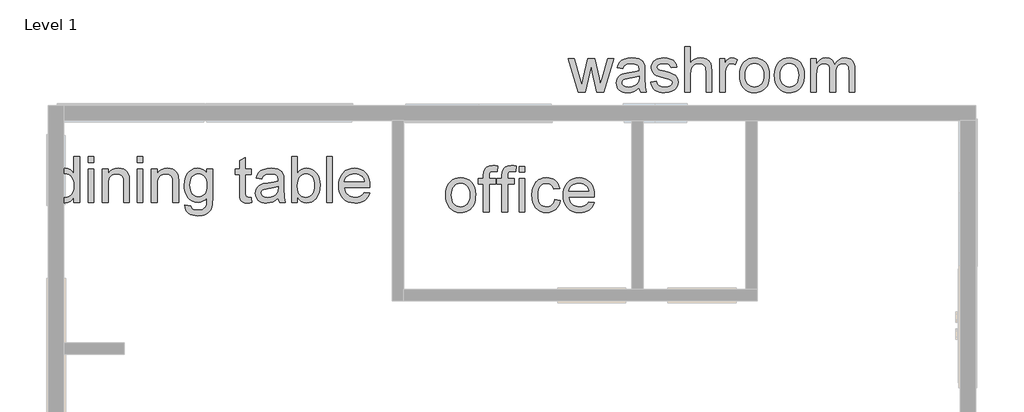
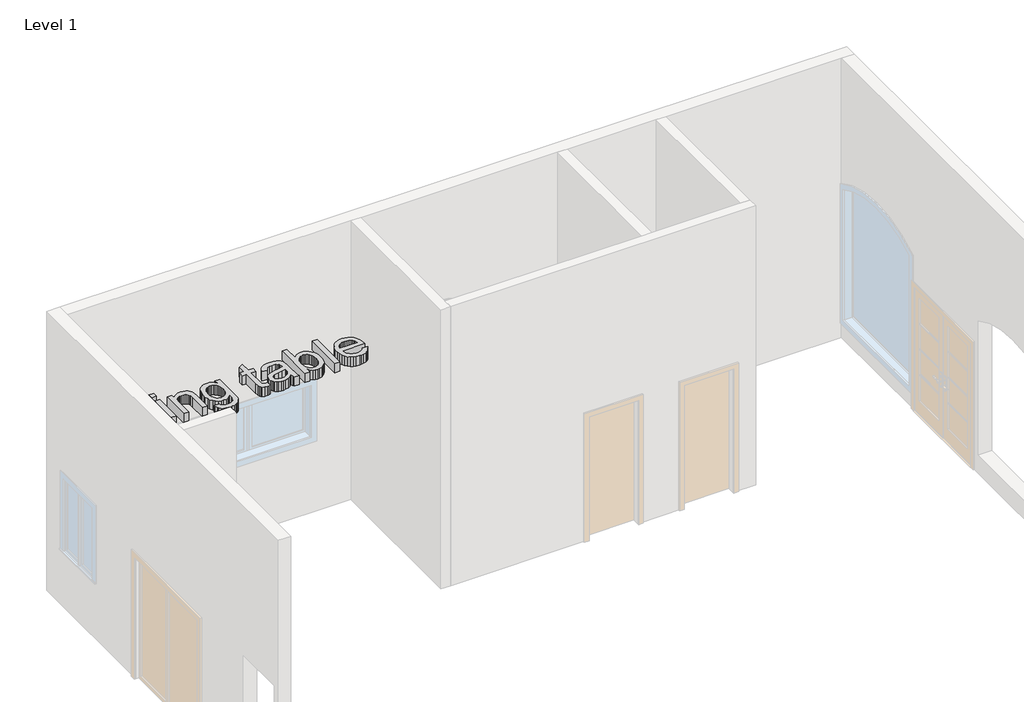
# One storey, part 3 of 3: 3 proxies.
"""IFC4 building model written with IfcOpenShell, lengths in millimetres."""

from ifc_helpers import new_model, si_unit, origin, origin_with_axes, place, context, project, spatial, polyline, outline, extrude, element, save

model = new_model("IFC4")

# Units and contexts
model_context = context("Model", 3, world=origin())
ifc_project = project(units=[si_unit("LENGTHUNIT", "METRE", prefix="MILLI")], contexts=[model_context])

# Site, building, storey
site = spatial("IfcSite", under=ifc_project)
building = spatial("IfcBuilding", under=site)
storey = spatial("IfcBuildingStorey", under=building, Name="Level 1", Elevation=0.0)

# Proxies
placement = place(None, origin())
element("IfcBuildingElementProxy", 1, Name="24\" Arial", ObjectType="24\" Arial", at=placement, inside=storey, context=model_context, shape_type="SweptSolid", body=[
    extrude(outline(polyline([(-71376.3912877, -6229.4340797), (-71512.4649649, -5782.1011603), (-71433.3489034, -5782.1011603), (-71356.1661291, -6043.0949348), (-71333.1153968, -6136.3388645), (-71314.2286679, -6046.515366), (-71252.8096201, -5782.1011603), (-71162.0938352, -5782.1011603), (-71100.9722163, -6045.771794), (-71084.1674889, -6127.1185716), (-71060.0757559, -6041.310362), (-70982.7442671, -5782.1011603), (-70903.3307768, -5782.1011603), (-71040.4454549, -6229.4340797), (-71132.4996694, -6229.4340797), (-71190.9444291, -5967.1018757), (-71207.8978709, -5885.3089549), (-71283.2960724, -6229.4340797), (-71376.3912877, -6229.4340797)])), origin_with_axes(), (0.0, 0.0, 1.0), 152.4),
    extrude(outline(polyline([(-70565.4516568, -6172.3277496), (-70601.8309173, -6203.5205953), (-70639.2883571, -6223.9316469), (-70678.6790842, -6235.1967628), (-70720.8582063, -6238.9518014), (-70754.7604425, -6236.6932015), (-70784.4893808, -6229.9174015), (-70810.0450212, -6218.6244017), (-70831.4273637, -6202.8142019), (-70848.3110956, -6183.4906244), (-70860.3709041, -6161.6574913), (-70867.6067892, -6137.3148027), (-70870.0187509, -6110.4625586), (-70866.3752481, -6078.8979269), (-70855.4447395, -6050.2332261), (-70838.5842443, -6025.6953498), (-70817.1507812, -6006.511192), (-70791.9622795, -5992.0115379), (-70763.8366683, -5981.5271726), (-70697.9561885, -5970.0761637), (-70620.1041993, -5958.0302972), (-70565.8978, -5943.902429), (-70565.4516568, -5926.9489873), (-70570.6938395, -5892.9677466), (-70577.2465678, -5880.3827904), (-70586.4203874, -5870.7349436), (-70602.2770605, -5861.1056861), (-70621.5913433, -5854.227645), (-70670.5927386, -5848.7252122), (-70715.950631, -5852.3873043), (-70747.6267985, -5863.3735807), (-70769.2275653, -5883.6916858), (-70784.3592557, -5915.349264), (-70860.5010292, -5905.8315423), (-70847.2840368, -5864.1915099), (-70827.5607893, -5831.4743416), (-70799.490946, -5806.4531436), (-70761.2341663, -5787.901022), (-70714.4448977, -5776.4128345), (-70660.7775881, -5772.5834386), (-70609.3038159, -5775.9666913), (-70568.500302, -5786.1164492), (-70537.7350103, -5801.3782646), (-70516.3759044, -5820.0976899), (-70502.2108576, -5843.2413686), (-70493.0277433, -5871.7759444), (-70489.3098833, -5938.3999962), (-70489.3098833, -6033.1310699), (-70485.4433089, -6165.4125299), (-70479.7178044, -6198.1111089), (-70470.2744399, -6229.4340797), (-70546.4162134, -6229.4340797), (-70558.6107944, -6202.9629163), (-70565.4516568, -6172.3277496)]), holes=[polyline([(-70565.4516568, -6020.0442026), (-70616.6094109, -6032.7221053), (-70688.2897524, -6043.3923636), (-70753.7984462, -6055.7356589), (-70770.8448345, -6064.1752012), (-70783.4669693, -6075.8121031), (-70791.2744753, -6089.7540782), (-70793.8769774, -6105.1088402), (-70788.2072408, -6127.7506078), (-70771.1980312, -6146.3027294), (-70743.2211344, -6158.6832033), (-70704.6483365, -6162.8100279), (-70663.7518761, -6158.2556494), (-70627.6142766, -6144.5925137), (-70598.3175395, -6124.4603017), (-70577.9436665, -6100.4986937), (-70568.9092666, -6075.8121031), (-70565.8978, -6041.6077908), (-70565.4516568, -6020.0442026)])]), origin_with_axes(), (0.0, 0.0, 1.0), 152.4),
    extrude(outline(polyline([(-70413.1681098, -6096.1859761), (-70337.0263363, -6086.6682544), (-70332.4254845, -6104.0306608), (-70325.0176484, -6119.2367083), (-70314.8028279, -6132.286397), (-70301.7810231, -6143.1797269), (-70285.9150554, -6151.7679836), (-70267.1677462, -6157.9024527), (-70221.0291032, -6162.8100279), (-70175.4481391, -6158.3114173), (-70157.7325361, -6152.688154), (-70143.4001856, -6144.8155853), (-70124.4390995, -6125.2596416), (-70119.6988279, -6114.3105438), (-70118.1187374, -6102.5806953), (-70119.7081226, -6092.3008123), (-70124.4762781, -6083.173466), (-70143.5489, -6068.376383), (-70172.0648865, -6058.7099469), (-70221.9213896, -6046.6640804), (-70291.4081936, -6026.5690469), (-70336.5801931, -6009.4111229), (-70365.5980906, -5990.6916976), (-70386.6225891, -5965.9121605), (-70399.3934384, -5936.652602), (-70403.6503881, -5904.4931127), (-70400.2299569, -5874.9918933), (-70389.9686632, -5847.7585685), (-70373.795972, -5823.8713178), (-70352.6413484, -5804.4083205), (-70331.6168499, -5792.1579717), (-70304.2348108, -5781.8780887), (-70272.5772326, -5774.9071012), (-70238.7261169, -5772.5834386), (-70189.1670427, -5776.319888), (-70146.0770449, -5787.529236), (-70111.4265893, -5805.1147139), (-70087.1861419, -5827.9795532), (-70071.1249866, -5857.8153799), (-70061.0124073, -5896.3138206), (-70137.1541808, -5905.8315423), (-70146.764849, -5881.8699344), (-70165.7817031, -5863.8197239), (-70194.390636, -5852.4988401), (-70232.7775409, -5848.7252122), (-70276.4995749, -5852.3315364), (-70305.6475976, -5863.1505091), (-70322.0433603, -5878.7655212), (-70327.5086146, -5896.7599638), (-70325.24072, -5908.4712229), (-70318.4370361, -5918.9184096), (-70306.8001342, -5928.2502383), (-70290.0325854, -5935.723137), (-70224.4495344, -5951.9330067), (-70157.1748571, -5971.8235579), (-70112.6906618, -5987.7731775), (-70083.1708531, -6004.9125122), (-70060.7893357, -6028.372209), (-70046.6800568, -6058.2266251), (-70041.9769639, -6094.5501177), (-70047.497986, -6132.100504), (-70064.0610525, -6167.4201744), (-70091.034127, -6197.7393229), (-70127.7851735, -6220.2881441), (-70172.1764223, -6234.2858871), (-70222.070104, -6238.9518014), (-70263.0502162, -6236.7024961), (-70298.8439137, -6229.9545801), (-70329.4511964, -6218.7080535), (-70354.8720644, -6202.9629163), (-70375.6363127, -6182.7935256), (-70392.2737364, -6158.2742387), (-70404.7843354, -6129.4050555), (-70413.1681098, -6096.1859761)])), origin_with_axes(), (0.0, 0.0, 1.0), 152.4),
    extrude(outline(polyline([(-69956.3174687, -6229.4340797), (-69956.3174687, -5620.2998916), (-69880.1756952, -5620.2998916), (-69880.1756952, -5844.2637801), (-69852.2080931, -5812.9036307), (-69820.8014704, -5790.503524), (-69785.9558272, -5777.06346), (-69747.6711635, -5772.5834386), (-69701.6812349, -5777.4724246), (-69662.1603827, -5792.1393824), (-69631.0418942, -5815.4317755), (-69619.3585191, -5829.8803091), (-69610.2590566, -5846.1970673), (-69598.5477975, -5888.4691359), (-69594.6440445, -5946.2818595), (-69594.6440445, -6229.4340797), (-69670.785818, -6229.4340797), (-69670.785818, -5954.1637227), (-69672.300846, -5928.4547206), (-69676.8459298, -5906.5007571), (-69684.4210697, -5888.3018322), (-69695.0262654, -5873.857946), (-69708.4105615, -5862.8623749), (-69724.3230025, -5855.0083956), (-69742.7635883, -5850.296008), (-69763.7323189, -5848.7252122), (-69795.9103975, -5852.9635726), (-69826.1180103, -5865.6786539), (-69851.1392083, -5885.6435623), (-69867.7580426, -5911.6314039), (-69877.071282, -5946.1703237), (-69880.1756952, -5991.7884663), (-69880.1756952, -6229.4340797), (-69956.3174687, -6229.4340797)])), origin_with_axes(), (0.0, 0.0, 1.0), 152.4),
    extrude(outline(polyline([(-69489.9491059, -6229.4340797), (-69489.9491059, -5782.1011603), (-69423.3250541, -5782.1011603), (-69423.3250541, -5848.2790689), (-69398.7128206, -5809.9107534), (-69376.0338744, -5787.3061644), (-69353.280571, -5776.2641201), (-69328.445266, -5772.5834386), (-69290.5230936, -5778.4576575), (-69252.0060636, -5796.0803141), (-69277.4362263, -5864.3402243), (-69304.2048185, -5852.6289652), (-69330.9734108, -5848.7252122), (-69353.7081249, -5852.4802508), (-69374.02623, -5863.7453667), (-69390.4405821, -5881.6654521), (-69401.4640371, -5905.3853991), (-69410.7215085, -5947.9177179), (-69413.8073324, -5994.3166111), (-69413.8073324, -6229.4340797), (-69489.9491059, -6229.4340797)])), origin_with_axes(), (0.0, 0.0, 1.0), 152.4),
    extrude(outline(polyline([(-69223.4528986, -6005.76762), (-69219.3353686, -5947.834066), (-69206.9827786, -5897.9125004), (-69186.3951287, -5856.0029232), (-69157.5724188, -5822.1053343), (-69128.5545212, -5800.4395049), (-69096.525157, -5784.9639126), (-69061.4843262, -5775.6785571), (-69023.4320287, -5772.5834386), (-68981.4248576, -5776.3524192), (-68943.44227, -5787.6593611), (-68909.4842659, -5806.5042641), (-68879.5508453, -5832.8871284), (-68855.1198576, -5865.9156675), (-68837.669152, -5904.697595), (-68827.1987287, -5949.2329109), (-68823.7085876, -5999.5216152), (-68825.2514995, -6040.2786558), (-68829.8802353, -6076.4441393), (-68837.5947948, -6108.0180656), (-68848.3951782, -6135.0004348), (-68862.1466131, -6158.3067699), (-68878.7143268, -6178.852594), (-68898.0983196, -6196.6379069), (-68920.2985913, -6211.6627088), (-68944.4507396, -6223.6016868), (-68969.6903619, -6232.1295283), (-68996.0174583, -6237.2462331), (-69023.4320287, -6238.9518014), (-69066.0526467, -6235.1967628), (-69104.388431, -6223.9316469), (-69138.4393816, -6205.1564537), (-69168.2054985, -6178.8711833), (-69192.376236, -6145.5219787), (-69209.6410485, -6105.5549834), (-69219.9999361, -6058.9701971), (-69223.4528986, -6005.76762)]), holes=[polyline([(-69147.3111251, -6005.6189056), (-69145.108293, -6042.5511978), (-69138.4997968, -6074.5294414), (-69127.4856364, -6101.5536365), (-69112.0658119, -6123.6237831), (-69093.3092081, -6140.7677652), (-69072.2847096, -6153.0134667), (-69048.9923164, -6160.3608876), (-69023.4320287, -6162.8100279), (-68998.0018661, -6160.3469456), (-68974.8024194, -6152.9576988), (-68953.8336888, -6140.6422875), (-68935.0956743, -6123.4007115), (-68919.6758498, -6101.1121406), (-68908.6616894, -6073.6557443), (-68902.0531932, -6041.0315225), (-68899.8503611, -6003.2394752), (-68902.0671352, -5967.478309), (-68908.7174573, -5936.3365839), (-68919.8013275, -5909.8142999), (-68935.3187459, -5887.9114569), (-68954.1264703, -5870.7674748), (-68975.0812589, -5858.5217733), (-68998.1831117, -5851.1743525), (-69023.4320287, -5848.7252122), (-69048.9923164, -5851.1650578), (-69072.2847096, -5858.4845947), (-69093.3092081, -5870.683823), (-69112.0658119, -5887.7627425), (-69127.4856364, -5909.7678266), (-69138.4997968, -5936.7455485), (-69145.108293, -5968.6959082), (-69147.3111251, -6005.6189056)])]), origin_with_axes(), (0.0, 0.0, 1.0), 152.4),
    extrude(outline(polyline([(-68757.0845358, -6005.76762), (-68752.9670058, -5947.834066), (-68740.6144158, -5897.9125004), (-68720.0267659, -5856.0029232), (-68691.204056, -5822.1053343), (-68662.1861584, -5800.4395049), (-68630.1567942, -5784.9639126), (-68595.1159634, -5775.6785571), (-68557.0636659, -5772.5834386), (-68515.0564948, -5776.3524192), (-68477.0739072, -5787.6593611), (-68443.1159032, -5806.5042641), (-68413.1824825, -5832.8871284), (-68388.7514948, -5865.9156675), (-68371.3007893, -5904.697595), (-68360.8303659, -5949.2329109), (-68357.3402248, -5999.5216152), (-68358.8831367, -6040.2786558), (-68363.5118725, -6076.4441393), (-68371.2264321, -6108.0180656), (-68382.0268155, -6135.0004348), (-68395.7782503, -6158.3067699), (-68412.345964, -6178.852594), (-68431.7299568, -6196.6379069), (-68453.9302285, -6211.6627088), (-68478.0823768, -6223.6016868), (-68503.3219991, -6232.1295283), (-68529.6490955, -6237.2462331), (-68557.0636659, -6238.9518014), (-68599.6842839, -6235.1967628), (-68638.0200682, -6223.9316469), (-68672.0710188, -6205.1564537), (-68701.8371357, -6178.8711833), (-68726.0078732, -6145.5219787), (-68743.2726858, -6105.5549834), (-68753.6315733, -6058.9701971), (-68757.0845358, -6005.76762)]), holes=[polyline([(-68680.9427623, -6005.6189056), (-68678.7399302, -6042.5511978), (-68672.131434, -6074.5294414), (-68661.1172736, -6101.5536365), (-68645.6974491, -6123.6237831), (-68626.9408453, -6140.7677652), (-68605.9163468, -6153.0134667), (-68582.6239536, -6160.3608876), (-68557.0636659, -6162.8100279), (-68531.6335033, -6160.3469456), (-68508.4340566, -6152.9576988), (-68487.465326, -6140.6422875), (-68468.7273115, -6123.4007115), (-68453.307487, -6101.1121406), (-68442.2933266, -6073.6557443), (-68435.6848304, -6041.0315225), (-68433.4819983, -6003.2394752), (-68435.6987724, -5967.478309), (-68442.3490945, -5936.3365839), (-68453.4329648, -5909.8142999), (-68468.9503831, -5887.9114569), (-68487.7581075, -5870.7674748), (-68508.7128961, -5858.5217733), (-68531.8147489, -5851.1743525), (-68557.0636659, -5848.7252122), (-68582.6239536, -5851.1650578), (-68605.9163468, -5858.4845947), (-68626.9408453, -5870.683823), (-68645.6974491, -5887.7627425), (-68661.1172736, -5909.7678266), (-68672.131434, -5936.7455485), (-68678.7399302, -5968.6959082), (-68680.9427623, -6005.6189056)])]), origin_with_axes(), (0.0, 0.0, 1.0), 152.4),
    extrude(outline(polyline([(-68271.6807296, -6229.4340797), (-68271.6807296, -5782.1011603), (-68195.5389561, -5782.1011603), (-68195.5389561, -5855.714789), (-68172.6369383, -5821.900852), (-68143.1914868, -5795.4110993), (-68108.2064239, -5778.2903538), (-68068.6855717, -5772.5834386), (-68026.3391459, -5778.4018896), (-68008.3168194, -5785.6749533), (-67992.3950838, -5795.8572425), (-67978.6204124, -5808.660623), (-67967.0392783, -5823.7969606), (-67950.4576226, -5861.0685075), (-67922.7037974, -5822.3562899), (-67891.0462192, -5794.7047058), (-67855.484888, -5778.1137554), (-67816.0198037, -5772.5834386), (-67785.5379988, -5774.8838645), (-67758.7833485, -5781.7851422), (-67735.7558529, -5793.2872717), (-67716.455512, -5809.390253), (-67701.1983439, -5830.2799791), (-67690.3003666, -5856.1423429), (-67683.7615803, -5886.9773446), (-67681.5819849, -5922.7849841), (-67681.5819849, -6229.4340797), (-67757.7237584, -6229.4340797), (-67757.7237584, -5955.5021524), (-67759.4897419, -5917.5242121), (-67764.7876924, -5891.9267458), (-67774.7143787, -5874.3970357), (-67790.3665695, -5860.6223643), (-67810.4987816, -5851.6995002), (-67833.8655319, -5848.7252122), (-67855.4430621, -5850.6306154), (-67875.115189, -5856.3468252), (-67892.8819126, -5865.8738416), (-67908.743233, -5879.2116644), (-67921.7882744, -5896.7506692), (-67931.1061611, -5918.881231), (-67936.6968931, -5945.60335), (-67938.5604705, -5976.9170262), (-67938.5604705, -6229.4340797), (-68014.702244, -6229.4340797), (-68014.702244, -5947.0254315), (-68019.1079081, -5903.9726123), (-68024.6149883, -5887.0749384), (-68032.3249006, -5873.2630884), (-68042.5443683, -5862.5277675), (-68055.5801151, -5854.8596812), (-68071.4321408, -5850.2588294), (-68090.1004455, -5848.7252122), (-68119.4343612, -5852.8148582), (-68146.4632036, -5865.0837963), (-68168.7703638, -5885.2345977), (-68183.9392328, -5912.9698336), (-68192.6390253, -5951.4496849), (-68195.5389561, -6003.8343328), (-68195.5389561, -6229.4340797), (-68271.6807296, -6229.4340797)])), origin_with_axes(), (0.0, 0.0, 1.0), 152.4),
])
element("IfcBuildingElementProxy", 2, Name="24\" Arial", ObjectType="24\" Arial", at=placement, inside=storey, context=model_context, shape_type="SweptSolid", body=[
    extrude(outline(polyline([(-73151.8600009, -7609.8505265), (-73147.742471, -7551.9169725), (-73135.389881, -7501.9954069), (-73114.802231, -7460.0858296), (-73085.9795211, -7426.1882408), (-73056.9616235, -7404.5224114), (-73024.9322593, -7389.046819), (-72989.8914285, -7379.7614636), (-72951.8391311, -7376.6663451), (-72909.83196, -7380.4353257), (-72871.8493724, -7391.7422675), (-72837.8913683, -7410.5871706), (-72807.9579477, -7436.9700349), (-72783.5269599, -7469.998574), (-72766.0762544, -7508.7805014), (-72755.6058311, -7553.3158173), (-72752.11569, -7603.6045216), (-72753.6586019, -7644.3615623), (-72758.2873376, -7680.5270458), (-72766.0018972, -7712.1009721), (-72776.8022806, -7739.0833413), (-72790.5537154, -7762.3896764), (-72807.1214292, -7782.9355004), (-72826.505422, -7800.7208134), (-72848.7056937, -7815.7456152), (-72872.8578419, -7827.6845933), (-72898.0974642, -7836.2124347), (-72924.4245606, -7841.3291396), (-72951.8391311, -7843.0347079), (-72994.459749, -7839.2796693), (-73032.7955333, -7828.0145534), (-73066.8464839, -7809.2393602), (-73096.6126008, -7782.9540897), (-73120.7833384, -7749.6048852), (-73138.0481509, -7709.6378898), (-73148.4070384, -7663.0531036), (-73151.8600009, -7609.8505265)]), holes=[polyline([(-73075.7182274, -7609.7018121), (-73073.5153954, -7646.6341042), (-73066.9068991, -7678.6123478), (-73055.8927388, -7705.636543), (-73040.4729143, -7727.7066896), (-73021.7163104, -7744.8506717), (-73000.6918119, -7757.0963732), (-72977.3994188, -7764.4437941), (-72951.8391311, -7766.8929344), (-72926.4089684, -7764.4298521), (-72903.2095218, -7757.0406053), (-72882.2407912, -7744.7251939), (-72863.5027766, -7727.483618), (-72848.0829521, -7705.1950471), (-72837.0687918, -7677.7386507), (-72830.4602956, -7645.1144289), (-72828.2574635, -7607.3223817), (-72830.4742375, -7571.5612155), (-72837.1245597, -7540.4194903), (-72848.2084299, -7513.8972063), (-72863.7258482, -7491.9943634), (-72882.5335727, -7474.8503813), (-72903.4883613, -7462.6046798), (-72926.5902141, -7455.2572589), (-72951.8391311, -7452.8081186), (-72977.3994188, -7455.2479643), (-73000.6918119, -7462.5675012), (-73021.7163104, -7474.7667295), (-73040.4729143, -7491.845649), (-73055.8927388, -7513.8507331), (-73066.9068991, -7540.8284549), (-73073.5153954, -7572.7788146), (-73075.7182274, -7609.7018121)])]), origin_with_axes(), (0.0, 0.0, 1.0), 152.4),
    extrude(outline(polyline([(-72647.4207514, -7833.5169862), (-72647.4207514, -7462.3258403), (-72714.0448032, -7462.3258403), (-72714.0448032, -7386.1840668), (-72647.4207514, -7386.1840668), (-72647.4207514, -7341.1236032), (-72645.413107, -7303.833467), (-72639.3901737, -7277.6225538), (-72624.0725904, -7252.3039269), (-72600.4270005, -7232.2646613), (-72567.3380462, -7219.2149726), (-72523.6903694, -7214.8650764), (-72490.6385937, -7216.947078), (-72454.240744, -7223.1930829), (-72465.3943241, -7294.5759955), (-72509.2650725, -7291.0068499), (-72538.2086129, -7294.1670309), (-72557.2254669, -7303.647574), (-72567.7656001, -7321.7535524), (-72571.2789779, -7350.7900393), (-72571.2789779, -7386.1840668), (-72485.6194827, -7386.1840668), (-72485.6194827, -7462.3258403), (-72571.2789779, -7462.3258403), (-72571.2789779, -7833.5169862), (-72647.4207514, -7833.5169862)])), origin_with_axes(), (0.0, 0.0, 1.0), 152.4),
    extrude(outline(polyline([(-72399.9599875, -7833.5169862), (-72399.9599875, -7462.3258403), (-72466.5840393, -7462.3258403), (-72466.5840393, -7386.1840668), (-72399.9599875, -7386.1840668), (-72399.9599875, -7341.1236032), (-72397.952343, -7303.833467), (-72391.9294098, -7277.6225538), (-72376.6118264, -7252.3039269), (-72352.9662366, -7232.2646613), (-72319.8772823, -7219.2149726), (-72276.2296055, -7214.8650764), (-72243.1778298, -7216.947078), (-72206.77998, -7223.1930829), (-72217.9335601, -7294.5759955), (-72261.8043086, -7291.0068499), (-72290.7478489, -7294.1670309), (-72309.764703, -7303.647574), (-72320.3048362, -7321.7535524), (-72323.8182139, -7350.7900393), (-72323.8182139, -7386.1840668), (-72238.1587187, -7386.1840668), (-72238.1587187, -7462.3258403), (-72323.8182139, -7462.3258403), (-72323.8182139, -7833.5169862), (-72399.9599875, -7833.5169862)])), origin_with_axes(), (0.0, 0.0, 1.0), 152.4),
    extrude(outline(polyline([(-72171.5346669, -7833.5169862), (-72171.5346669, -7386.1840668), (-72095.3928934, -7386.1840668), (-72095.3928934, -7833.5169862), (-72171.5346669, -7833.5169862)])), origin_with_axes(), (0.0, 0.0, 1.0), 152.4),
    extrude(outline(polyline([(-72171.5346669, -7300.5245716), (-72171.5346669, -7224.3827981), (-72095.3928934, -7224.3827981), (-72095.3928934, -7300.5245716), (-72171.5346669, -7300.5245716)])), origin_with_axes(), (0.0, 0.0, 1.0), 152.4),
    extrude(outline(polyline([(-71695.6485824, -7671.7157175), (-71619.5068089, -7681.2334392), (-71627.7883421, -7717.1619091), (-71640.7357897, -7748.9542597), (-71658.3491516, -7776.610491), (-71680.6284279, -7800.1306031), (-71706.6348588, -7818.9011489), (-71735.4296848, -7832.3086817), (-71767.0129058, -7840.3532013), (-71801.3845218, -7843.0347079), (-71844.0887916, -7839.2936112), (-71882.3781027, -7828.0703213), (-71916.2524549, -7809.364838), (-71945.7118484, -7783.1771613), (-71969.5572732, -7749.9999078), (-71986.5897195, -7710.3256939), (-71996.8091872, -7664.1545196), (-72000.2156765, -7611.4863849), (-71994.3972255, -7543.7283858), (-71987.1241618, -7513.2372862), (-71976.9418727, -7485.0047865), (-71963.7806482, -7459.5978605), (-71947.5707784, -7437.5834818), (-71928.3122634, -7418.9616503), (-71906.0051032, -7403.7323662), (-71881.6577673, -7391.8909819), (-71856.2787252, -7383.4328504), (-71829.867977, -7378.3579714), (-71802.4255226, -7376.6663451), (-71768.6441169, -7378.9900076), (-71738.0879547, -7385.9609952), (-71710.7570361, -7397.5793078), (-71686.6513611, -7413.8449455), (-71666.1798943, -7434.3861221), (-71649.7516003, -7458.8310519), (-71637.3664791, -7487.1797346), (-71629.0245306, -7519.4321704), (-71705.1663041, -7528.9498921), (-71718.9781541, -7495.7308127), (-71740.4859744, -7471.9179192), (-71768.5000498, -7457.5855688), (-71801.830665, -7452.8081186), (-71827.7023235, -7455.1596651), (-71851.0365426, -7462.2143045), (-71871.8333222, -7473.9720369), (-71890.0926623, -7490.4328622), (-71904.9594551, -7511.9778611), (-71915.5785928, -7538.9881142), (-71921.9500754, -7571.4636216), (-71924.073903, -7609.4043833), (-71921.9965487, -7647.9167659), (-71915.7644858, -7680.7687067), (-71905.3777143, -7707.9602055), (-71890.8362343, -7729.4912624), (-71872.9393855, -7745.8544939), (-71852.486508, -7757.5425164), (-71829.4776017, -7764.5553299), (-71803.9126666, -7766.8929344), (-71764.484761, -7761.0558941), (-71747.4337254, -7753.7595938), (-71732.157968, -7743.5447734), (-71719.0850426, -7730.299897), (-71708.6425032, -7713.9134289), (-71700.8303498, -7694.385369), (-71695.6485824, -7671.7157175)])), origin_with_axes(), (0.0, 0.0, 1.0), 152.4),
    extrude(outline(polyline([(-71239.6902277, -7700.2688826), (-71165.0355982, -7709.7866042), (-71176.4819598, -7739.6874936), (-71191.9343156, -7766.0378266), (-71211.3926655, -7788.8376032), (-71234.8570097, -7808.0868236), (-71262.0856871, -7823.376523), (-71292.8370369, -7834.2977368), (-71327.1110591, -7840.8504651), (-71364.9077537, -7843.0347079), (-71412.1524601, -7839.2657273), (-71454.2479304, -7827.9587855), (-71491.1941644, -7809.1138824), (-71522.9911624, -7782.7310181), (-71548.5607448, -7749.54447), (-71566.8247322, -7710.2885153), (-71577.7831247, -7664.9631542), (-71581.4359221, -7613.5683865), (-71577.7459461, -7560.430872), (-71566.6760178, -7513.5951302), (-71548.2261374, -7473.0611612), (-71522.3963048, -7438.8289649), (-71490.6829587, -7411.6328187), (-71454.5825378, -7392.207), (-71414.095042, -7380.5515088), (-71369.2204714, -7376.6663451), (-71325.7912188, -7380.5422142), (-71286.5166749, -7392.1698214), (-71251.3968395, -7411.5491669), (-71220.4317127, -7438.6802505), (-71195.1549118, -7472.8380896), (-71177.100054, -7513.2977014), (-71166.2671394, -7560.059086), (-71162.6561678, -7613.1222433), (-71163.102311, -7633.6448307), (-71505.2941486, -7633.6448307), (-71500.8838372, -7664.0290419), (-71492.1143348, -7690.6396251), (-71478.9856416, -7713.4765803), (-71461.4977574, -7732.5399077), (-71440.617326, -7747.5693568), (-71417.3109909, -7758.3046777), (-71391.5787521, -7764.7458702), (-71363.4206097, -7766.8929344), (-71322.8959353, -7762.9148241), (-71288.7659802, -7750.9804934), (-71261.0307443, -7730.3463702), (-71239.6902277, -7700.2688826)]), holes=[polyline([(-71505.2941486, -7557.5030572), (-71238.7979413, -7557.5030572), (-71249.0964136, -7517.2758116), (-71257.9542152, -7501.4563172), (-71269.2843936, -7488.499575), (-71290.0486419, -7472.8845628), (-71313.6756424, -7461.7309827), (-71340.1653952, -7455.0388346), (-71369.5179002, -7452.8081186), (-71396.2911397, -7454.5880441), (-71420.8429579, -7459.9278206), (-71443.1733548, -7468.827448), (-71463.2823302, -7481.2869265), (-71480.1567675, -7496.7299876), (-71492.7835496, -7514.5803631), (-71501.1626767, -7534.838053), (-71505.2941486, -7557.5030572)])]), origin_with_axes(), (0.0, 0.0, 1.0), 152.4),
])
element("IfcBuildingElementProxy", 3, Name="24\" Arial", ObjectType="24\" Arial", at=placement, inside=storey, context=model_context, shape_type="SweptSolid", body=[
    extrude(outline(polyline([(-78123.1451861, -7705.9587097), (-78123.1451861, -7634.1296538), (-78145.9263735, -7669.718869), (-78173.5221896, -7695.139737), (-78205.9326345, -7710.3922578), (-78243.1577081, -7715.4764314), (-78268.2904419, -7713.6360907), (-78292.3821749, -7708.1150685), (-78315.4329072, -7698.913365), (-78337.4426386, -7686.0309799), (-78357.7235651, -7669.8536415), (-78375.5878825, -7650.7670775), (-78391.035591, -7628.7712881), (-78404.0666904, -7603.8662732), (-78414.4116359, -7576.5260599), (-78421.8008828, -7547.2246755), (-78427.7122802, -7482.7383932), (-78422.2656153, -7419.0514508), (-78405.9256204, -7361.5361561), (-78393.6752716, -7335.9108058), (-78378.710885, -7313.4642258), (-78361.0324605, -7294.1964162), (-78340.6399982, -7278.1073769), (-78318.2538335, -7265.4201795), (-78294.5943017, -7256.3578957), (-78269.6614028, -7250.9205254), (-78243.4551369, -7249.1080686), (-78206.2021793, -7254.2944834), (-78173.2619394, -7269.8537276), (-78145.3408106, -7293.7037997), (-78123.1451861, -7323.7626981), (-78123.1451861, -7096.8245216), (-78047.0034126, -7096.8245216), (-78047.0034126, -7705.9587097), (-78123.1451861, -7705.9587097)]), holes=[polyline([(-78351.5705067, -7482.4409644), (-78349.4234425, -7519.3639619), (-78342.98225, -7551.3143216), (-78332.2469292, -7578.2920434), (-78317.21748, -7600.2971275), (-78299.2695107, -7617.3760471), (-78279.7786294, -7629.5752753), (-78258.7448363, -7636.8948122), (-78236.1681312, -7639.3346579), (-78213.4845377, -7637.006348), (-78192.5762223, -7630.0214185), (-78173.4431851, -7618.3798693), (-78156.0854261, -7602.0817003), (-78141.6740711, -7580.9967866), (-78131.3802461, -7554.995003), (-78125.2039511, -7524.0763495), (-78123.1451861, -7488.2408261), (-78125.2411297, -7448.9523402), (-78131.5289605, -7415.2592336), (-78142.0086785, -7387.1615064), (-78156.6802837, -7364.6591585), (-78174.4191234, -7347.4175826), (-78194.1005449, -7335.1021712), (-78215.7245483, -7327.7129244), (-78239.2911336, -7325.2498421), (-78262.3139819, -7327.6153306), (-78283.3477751, -7334.7117959), (-78302.3925131, -7346.5392382), (-78319.448196, -7363.0976573), (-78333.5017069, -7384.7495447), (-78343.539929, -7411.8573917), (-78349.5628623, -7444.4211982), (-78351.5705067, -7482.4409644)])]), origin_with_axes(), (0.0, 0.0, 1.0), 152.4),
    extrude(outline(polyline([(-77932.7907524, -7705.9587097), (-77932.7907524, -7258.6257903), (-77856.6489788, -7258.6257903), (-77856.6489788, -7705.9587097), (-77932.7907524, -7705.9587097)])), origin_with_axes(), (0.0, 0.0, 1.0), 152.4),
    extrude(outline(polyline([(-77932.7907524, -7172.9662951), (-77932.7907524, -7096.8245216), (-77856.6489788, -7096.8245216), (-77856.6489788, -7172.9662951), (-77932.7907524, -7172.9662951)])), origin_with_axes(), (0.0, 0.0, 1.0), 152.4),
    extrude(outline(polyline([(-77742.4363186, -7705.9587097), (-77742.4363186, -7258.6257903), (-77666.294545, -7258.6257903), (-77666.294545, -7321.0858389), (-77639.8419709, -7289.5955644), (-77608.0728569, -7267.1025112), (-77570.987203, -7253.6066793), (-77528.5850093, -7249.1080686), (-77491.0532123, -7252.7329822), (-77456.6815963, -7263.6077228), (-77428.0168954, -7280.3752715), (-77407.6058438, -7301.6786095), (-77393.7568152, -7327.4619689), (-77384.7781832, -7357.6695816), (-77380.7628944, -7431.2832103), (-77380.7628944, -7705.9587097), (-77456.9046679, -7705.9587097), (-77456.9046679, -7441.544504), (-77459.0982053, -7402.1723663), (-77465.6788176, -7374.1768802), (-77477.8176306, -7354.1190253), (-77496.6857702, -7338.5597811), (-77520.8704498, -7328.5773269), (-77548.9588823, -7325.2498421), (-77572.0793244, -7327.1180668), (-77593.5546135, -7332.7227408), (-77613.3847494, -7342.0638641), (-77631.5697323, -7355.1414368), (-77646.7618379, -7373.4426028), (-77657.6133419, -7398.4545062), (-77664.1242442, -7430.177147), (-77666.294545, -7468.6105251), (-77666.294545, -7705.9587097), (-77742.4363186, -7705.9587097)])), origin_with_axes(), (0.0, 0.0, 1.0), 152.4),
    extrude(outline(polyline([(-77276.0679558, -7705.9587097), (-77276.0679558, -7258.6257903), (-77199.9261823, -7258.6257903), (-77199.9261823, -7705.9587097), (-77276.0679558, -7705.9587097)])), origin_with_axes(), (0.0, 0.0, 1.0), 152.4),
    extrude(outline(polyline([(-77276.0679558, -7172.9662951), (-77276.0679558, -7096.8245216), (-77199.9261823, -7096.8245216), (-77199.9261823, -7172.9662951), (-77276.0679558, -7172.9662951)])), origin_with_axes(), (0.0, 0.0, 1.0), 152.4),
    extrude(outline(polyline([(-77085.713522, -7705.9587097), (-77085.713522, -7258.6257903), (-77009.5717485, -7258.6257903), (-77009.5717485, -7321.0858389), (-76983.1191743, -7289.5955644), (-76951.3500603, -7267.1025112), (-76914.2644065, -7253.6066793), (-76871.8622128, -7249.1080686), (-76834.3304157, -7252.7329822), (-76799.9587997, -7263.6077228), (-76771.2940988, -7280.3752715), (-76750.8830472, -7301.6786095), (-76737.0340186, -7327.4619689), (-76728.0553866, -7357.6695816), (-76724.0400978, -7431.2832103), (-76724.0400978, -7705.9587097), (-76800.1818713, -7705.9587097), (-76800.1818713, -7441.544504), (-76802.3754087, -7402.1723663), (-76808.956021, -7374.1768802), (-76821.094834, -7354.1190253), (-76839.9629737, -7338.5597811), (-76864.1476532, -7328.5773269), (-76892.2360858, -7325.2498421), (-76915.3565278, -7327.1180668), (-76936.8318169, -7332.7227408), (-76956.6619528, -7342.0638641), (-76974.8469357, -7355.1414368), (-76990.0390413, -7373.4426028), (-77000.8905453, -7398.4545062), (-77007.4014477, -7430.177147), (-77009.5717485, -7468.6105251), (-77009.5717485, -7705.9587097), (-77085.713522, -7705.9587097)])), origin_with_axes(), (0.0, 0.0, 1.0), 152.4),
    extrude(outline(polyline([(-76638.3806026, -7744.0295965), (-76562.238829, -7753.5473182), (-76553.8364654, -7777.3416224), (-76537.5522384, -7793.7002066), (-76505.5414635, -7806.4152879), (-76463.6411809, -7810.6536483), (-76418.9525033, -7805.8576089), (-76400.9022928, -7799.8625596), (-76385.7148346, -7791.4694905), (-76362.6641024, -7768.4187583), (-76348.5362342, -7737.6348772), (-76344.4094096, -7704.8805303), (-76343.3312302, -7648.8523796), (-76368.6684463, -7673.836399), (-76396.9427719, -7691.6821272), (-76428.1542069, -7702.3895641), (-76462.3027513, -7705.9587097), (-76504.0496722, -7701.8040011), (-76540.8053659, -7689.3398754), (-76572.5698326, -7668.5663324), (-76599.3430722, -7639.4833723), (-76620.585995, -7604.5912559), (-76635.7595112, -7566.390244), (-76644.863621, -7524.8803367), (-76647.8983243, -7480.061534), (-76642.4516593, -7418.5867183), (-76626.1116644, -7362.0566565), (-76614.0007354, -7336.5660786), (-76599.454608, -7314.1520299), (-76582.4732823, -7294.8145104), (-76563.0567583, -7278.5535201), (-76541.5164067, -7265.6711351), (-76518.1635983, -7256.4694315), (-76492.9983332, -7250.9484093), (-76466.0206113, -7249.1080686), (-76430.4128069, -7253.2720719), (-76398.0953085, -7265.7640816), (-76369.0681163, -7286.5840978), (-76343.3312302, -7315.7321204), (-76343.3312302, -7258.6257903), (-76267.1894567, -7258.6257903), (-76267.1894567, -7644.8370907), (-76272.3944607, -7734.0099637), (-76278.9007158, -7767.1779225), (-76288.0094729, -7792.7335629), (-76299.9391563, -7813.3444495), (-76314.9081902, -7831.6781468), (-76332.9165748, -7847.7346548), (-76353.9643099, -7861.5139736), (-76377.8376186, -7872.5746072), (-76404.3227241, -7880.4750598), (-76433.4196262, -7885.2153313), (-76465.1283249, -7886.7954218), (-76502.4324031, -7884.5693531), (-76535.9721479, -7877.891147), (-76565.7475595, -7866.7608036), (-76591.7586377, -7851.1783227), (-76612.7691942, -7831.1251151), (-76627.5430406, -7806.5825916), (-76636.0801767, -7777.550752), (-76638.3806026, -7744.0295965)]), holes=[polyline([(-76571.7565507, -7474.8565299), (-76569.7256697, -7512.5045101), (-76563.6330266, -7544.6965307), (-76553.4786213, -7571.4325917), (-76539.262454, -7592.7126931), (-76521.9790522, -7608.9457994), (-76502.6229434, -7620.5408754), (-76481.1941276, -7627.497921), (-76457.6926049, -7629.8169362), (-76434.4234484, -7627.511863), (-76413.0968737, -7620.5966433), (-76393.712881, -7609.0712772), (-76376.2714701, -7592.9357647), (-76361.8601151, -7571.8647929), (-76351.5662902, -7545.5330492), (-76345.3899952, -7513.9405336), (-76343.3312302, -7477.087246), (-76345.4504104, -7441.772223), (-76351.8079511, -7411.076641), (-76362.4038522, -7385.0005002), (-76377.2381137, -7363.5438005), (-76395.0559579, -7346.7901937), (-76414.6026071, -7334.8233317), (-76435.8780611, -7327.6432145), (-76458.8823201, -7325.2498421), (-76481.5008511, -7327.6060359), (-76502.3626932, -7334.6746173), (-76521.4678464, -7346.4555863), (-76538.8163108, -7362.9489429), (-76553.2276658, -7384.0803299), (-76563.5214908, -7409.77539), (-76569.6977857, -7440.0341234), (-76571.7565507, -7474.8565299)])]), origin_with_axes(), (0.0, 0.0, 1.0), 152.4),
    extrude(outline(polyline([(-75753.2324854, -7642.4576603), (-75743.7147637, -7708.1894257), (-75773.8666086, -7713.65468), (-75800.6723795, -7715.4764314), (-75837.2189436, -7712.3162504), (-75864.4708577, -7702.8357073), (-75883.7293727, -7688.2245174), (-75896.2957396, -7669.6723958), (-75903.2109592, -7637.8103353), (-75905.5160325, -7583.2693286), (-75905.5160325, -7334.7675638), (-75962.6223626, -7334.7675638), (-75962.6223626, -7258.6257903), (-75905.5160325, -7258.6257903), (-75905.5160325, -7149.9155629), (-75829.3742589, -7105.1525281), (-75829.3742589, -7258.6257903), (-75753.2324854, -7258.6257903), (-75753.2324854, -7334.7675638), (-75829.3742589, -7334.7675638), (-75829.3742589, -7581.0386125), (-75825.3589701, -7620.2992145), (-75812.34646, -7634.204011), (-75801.3601836, -7638.0519962), (-75786.3957969, -7639.3346579), (-75753.2324854, -7642.4576603)])), origin_with_axes(), (0.0, 0.0, 1.0), 152.4),
    extrude(outline(polyline([(-75391.5590612, -7648.8523796), (-75427.9383217, -7680.0452253), (-75465.3957615, -7700.4562769), (-75504.7864886, -7711.7213928), (-75546.9656107, -7715.4764314), (-75580.8678469, -7713.2178314), (-75610.5967852, -7706.4420315), (-75636.1524256, -7695.1490317), (-75657.5347681, -7679.3388319), (-75674.4185, -7660.0152543), (-75686.4783085, -7638.1821213), (-75693.7141936, -7613.8394327), (-75696.1261553, -7586.9871886), (-75692.4826525, -7555.4225569), (-75681.552144, -7526.757856), (-75664.6916487, -7502.2199798), (-75643.2581856, -7483.035822), (-75618.0696839, -7468.5361679), (-75589.9440727, -7458.0518026), (-75524.0635929, -7446.6007937), (-75446.2116037, -7434.5549272), (-75392.0052044, -7420.427059), (-75391.5590612, -7403.4736173), (-75396.8012439, -7369.4923766), (-75403.3539722, -7356.9074203), (-75412.5277918, -7347.2595735), (-75428.3844649, -7337.6303161), (-75447.6987478, -7330.752275), (-75496.700143, -7325.2498421), (-75542.0580354, -7328.9119343), (-75573.7342029, -7339.8982107), (-75595.3349697, -7360.2163158), (-75610.4666601, -7391.873894), (-75686.6084336, -7382.3561723), (-75673.3914412, -7340.7161399), (-75653.6681937, -7307.9989716), (-75625.5983504, -7282.9777735), (-75587.3415707, -7264.425652), (-75540.5523021, -7252.9374645), (-75486.8849925, -7249.1080686), (-75435.4112203, -7252.4913213), (-75394.6077065, -7262.6410791), (-75363.8424147, -7277.9028946), (-75342.4833088, -7296.6223199), (-75328.318262, -7319.7659986), (-75319.1351477, -7348.3005744), (-75315.4172877, -7414.9246262), (-75315.4172877, -7509.6556999), (-75311.5507133, -7641.9371599), (-75305.8252088, -7674.6357389), (-75296.3818443, -7705.9587097), (-75372.5236178, -7705.9587097), (-75384.7181988, -7679.4875463), (-75391.5590612, -7648.8523796)]), holes=[polyline([(-75391.5590612, -7496.5688326), (-75442.7168153, -7509.2467353), (-75514.3971568, -7519.9169936), (-75579.9058506, -7532.2602889), (-75596.9522389, -7540.6998312), (-75609.5743737, -7552.3367331), (-75617.3818797, -7566.2787082), (-75619.9843818, -7581.6334702), (-75614.3146452, -7604.2752378), (-75597.3054356, -7622.8273593), (-75569.3285388, -7635.2078333), (-75530.7557409, -7639.3346579), (-75489.8592805, -7634.7802794), (-75453.721681, -7621.1171437), (-75424.4249439, -7600.9849316), (-75404.0510709, -7577.0233237), (-75395.0166711, -7552.3367331), (-75392.0052044, -7518.1324208), (-75391.5590612, -7496.5688326)])]), origin_with_axes(), (0.0, 0.0, 1.0), 152.4),
    extrude(outline(polyline([(-75134.5805756, -7705.9587097), (-75210.7223491, -7705.9587097), (-75210.7223491, -7096.8245216), (-75134.5805756, -7096.8245216), (-75134.5805756, -7322.7216973), (-75109.5407883, -7290.5157348), (-75081.2664627, -7267.5114758), (-75049.7575989, -7253.7089204), (-75015.0141969, -7249.1080686), (-74975.7907735, -7253.2534826), (-74938.723709, -7265.6897244), (-74905.9321834, -7285.6360435), (-74879.5353772, -7312.3116892), (-74858.8454861, -7345.4564114), (-74843.1747061, -7384.8099599), (-74833.3037877, -7428.7364762), (-74830.0134815, -7475.600102), (-74833.4199708, -7529.6763762), (-74843.6394386, -7577.2463953), (-74860.6718848, -7618.3101594), (-74884.5173096, -7652.8676684), (-74913.1401846, -7680.2590022), (-74944.5049813, -7699.8242407), (-74978.6116998, -7711.5633837), (-75015.4603401, -7715.4764314), (-75051.3469841, -7710.4294364), (-75083.1625713, -7695.2884514), (-75110.9071018, -7670.0534764), (-75134.5805756, -7634.7245115), (-75134.5805756, -7705.9587097)]), holes=[polyline([(-75134.5805756, -7479.1692476), (-75129.3755716, -7542.670297), (-75122.8693165, -7566.7248514), (-75113.7605594, -7585.648759), (-75095.310679, -7609.1363398), (-75073.8679212, -7625.9131832), (-75049.4322862, -7635.9792892), (-75022.0037737, -7639.3346579), (-74999.231881, -7636.862281), (-74978.0586681, -7629.4451502), (-74958.484135, -7617.0832656), (-74940.5082818, -7599.7766271), (-74925.4788326, -7577.5717081), (-74914.7435117, -7550.5149817), (-74908.3023192, -7518.6064479), (-74906.1552551, -7481.8461068), (-74908.21402, -7444.388667), (-74914.390315, -7412.1734098), (-74924.68414, -7385.2003352), (-74939.095495, -7363.4694433), (-74956.42537, -7346.7483678), (-74975.4747554, -7334.8047424), (-74996.243651, -7327.6385672), (-75018.7320569, -7325.2498421), (-75041.5039496, -7327.7222191), (-75062.6771625, -7335.1393498), (-75082.2516956, -7347.5012344), (-75100.2275489, -7364.8078729), (-75115.2569981, -7386.7897204), (-75125.9923189, -7413.177232), (-75132.4335114, -7443.9704077), (-75134.5805756, -7479.1692476)])]), origin_with_axes(), (0.0, 0.0, 1.0), 152.4),
    extrude(outline(polyline([(-74744.3539863, -7705.9587097), (-74744.3539863, -7096.8245216), (-74668.2122128, -7096.8245216), (-74668.2122128, -7705.9587097), (-74744.3539863, -7705.9587097)])), origin_with_axes(), (0.0, 0.0, 1.0), 152.4),
    extrude(outline(polyline([(-74240.8070232, -7572.7106061), (-74166.1523937, -7582.2283278), (-74177.5987553, -7612.1292171), (-74193.051111, -7638.4795501), (-74212.509461, -7661.2793268), (-74235.9738051, -7680.5285471), (-74263.2024826, -7695.8182465), (-74293.9538324, -7706.7394603), (-74328.2278546, -7713.2921886), (-74366.0245492, -7715.4764314), (-74413.2692556, -7711.7074508), (-74455.3647258, -7700.400509), (-74492.3109599, -7681.5556059), (-74524.1079579, -7655.1727416), (-74549.6775402, -7621.9861935), (-74567.9415277, -7582.7302389), (-74578.8999201, -7537.4048777), (-74582.5527176, -7486.0101101), (-74578.8627415, -7432.8725955), (-74567.7928133, -7386.0368537), (-74549.3429328, -7345.5028847), (-74523.5131002, -7311.2706884), (-74491.7997541, -7284.0745423), (-74455.6993332, -7264.6487236), (-74415.2118374, -7252.9932324), (-74370.3372668, -7249.1080686), (-74326.9080143, -7252.9839377), (-74287.6334703, -7264.611545), (-74252.513635, -7283.9908904), (-74221.5485082, -7311.121974), (-74196.2717073, -7345.2798131), (-74178.2168495, -7385.7394249), (-74167.3839348, -7432.5008095), (-74163.7729633, -7485.5639668), (-74164.2191065, -7506.0865542), (-74506.4109441, -7506.0865542), (-74502.0006326, -7536.4707654), (-74493.2311303, -7563.0813486), (-74480.102437, -7585.9183038), (-74462.6145529, -7604.9816312), (-74441.7341215, -7620.0110804), (-74418.4277864, -7630.7464012), (-74392.6955476, -7637.1875937), (-74364.5374051, -7639.3346579), (-74324.0127308, -7635.3565477), (-74289.8827756, -7623.4222169), (-74262.1475398, -7602.7880938), (-74240.8070232, -7572.7106061)]), holes=[polyline([(-74506.4109441, -7429.9447807), (-74239.9147368, -7429.9447807), (-74250.2132091, -7389.7175351), (-74259.0710106, -7373.8980407), (-74270.4011891, -7360.9412985), (-74291.1654374, -7345.3262863), (-74314.7924379, -7334.1727062), (-74341.2821906, -7327.4805582), (-74370.6346956, -7325.2498421), (-74397.4079352, -7327.0297676), (-74421.9597534, -7332.3695441), (-74444.2901502, -7341.2691716), (-74464.3991257, -7353.72865), (-74481.2735629, -7369.1717111), (-74493.9003451, -7387.0220866), (-74502.2794721, -7407.2797765), (-74506.4109441, -7429.9447807)])]), origin_with_axes(), (0.0, 0.0, 1.0), 152.4),
])

save(model, "model.ifc")

# Revit data of these elements
# Project information
#   Project Issue Date = "Issue Date"
#   Project Status = "Project Status"
#   Client Name = "Owner"
#   Project Address = "Enter address here"
#   Project Name = "Project Name"
#   Project Number = "Project Number"
# Elements 1, 2, 3 (IfcBuildingElementProxy, "24\" Arial")
#   Phase Created = New Construction
